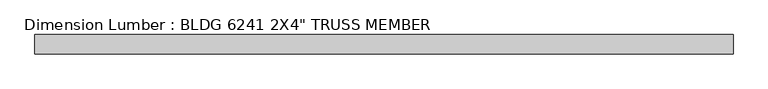
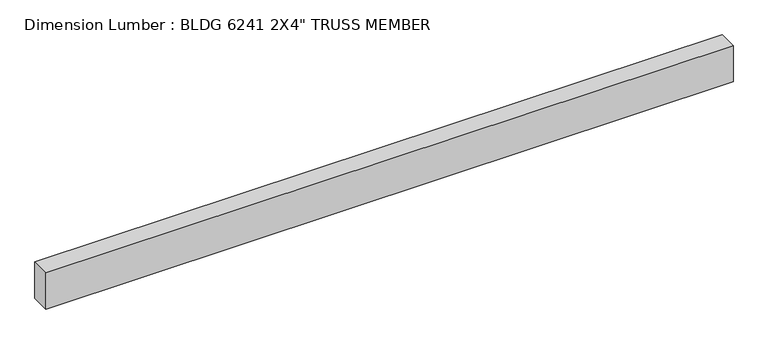
"""IFC4 building model written with IfcOpenShell, lengths in millimetres: beam geometry."""

from ifc_helpers import new_model, si_unit, frame, origin, place, context, project, spatial, polyline, outline, extrude, source, transform, mapped, element, save


def beam_17170791(model_context):
    return source(origin(), model_context, "Body", "SweptSolid", [
        extrude(outline(polyline([(914.3999994, 25.4), (914.3999994, -25.4), (-914.3999994, -25.4), (-914.3999994, 25.4), (914.3999994, 25.4)])), frame((0.0, 0.0, -50.8), z_axis=(0.0, 0.0, 1.0), x_axis=(1.0, 0.0, 0.0)), (0.0, 0.0, 1.0), 101.6),
    ])


if __name__ == "__main__":
    model = new_model("IFC4")
    model_context = context("Model", 3, world=origin())
    ifc_project = project(units=[si_unit("LENGTHUNIT", "METRE", prefix="MILLI")], contexts=[model_context])
    site = spatial("IfcSite", under=ifc_project)
    building = spatial("IfcBuilding", under=site)
    placement = place(None, origin())
    beam_shape = beam_17170791(model_context)
    element("IfcBeam", 1, ObjectType="Dimension Lumber : BLDG 6241 2X4\" TRUSS MEMBER", at=placement, inside=building, context=model_context, shape_type="MappedRepresentation", body=[
        mapped(beam_shape, transform((0.0, 0.0, 0.0), x_axis=(1.0, 0.0, 0.0), y_axis=(0.0, 1.0, 0.0), z_axis=(0.0, 0.0, 1.0))),
    ])
    save(model, "model.ifc")

# Revit data of these elements
# Type "Dimension Lumber : BLDG 6241 2X4\" TRUSS MEMBER"
#   Assembly Code = "B10"
#   A = 0.273472 SF
#   Length [instance default] = 5' - 0"
#   b = 0' - 2"
#   d = 0' - 4"
#   Structural Material [instance default] = Softwood, Lumber
# Element 1 (IfcBeam, "Dimension Lumber : BLDG 6241 2X4\" TRUSS MEMBER")
#   Materials on its faces: "Softwood, Lumber"
# Materials
#   "Softwood, Lumber": class "Wood", colour RGB 223 192 134, transparency 0, Description = "Pinus Echinata", Cost = 0
